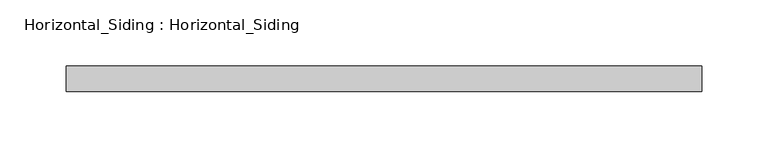
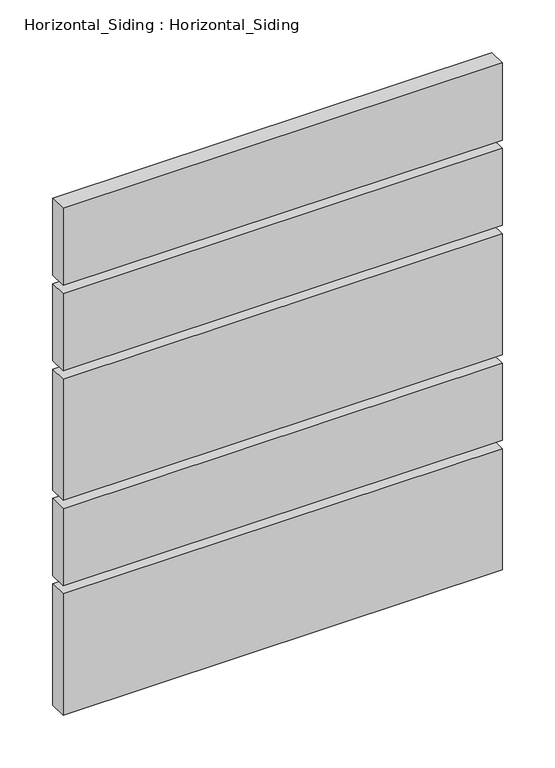
"""IFC4 building model written with IfcOpenShell, lengths in millimetres: plate geometry, Horizontal_Siding : Horizontal_Siding."""

from ifc_helpers import new_model, si_unit, frame, origin, place, context, project, spatial, polyline, outline, extrude, source, transform, mapped, element, save


def horizontal_siding_horizontal_siding_d49449ac(model_context):
    return source(origin(), model_context, "Body", "SweptSolid", [
        extrude(outline(polyline([(239.3754093, -19.05), (-239.3754093, -19.05), (-239.3754093, 0.0), (239.3754093, 0.0), (239.3754093, -19.05)])), frame((0.0, 0.0, 9.525), z_axis=(0.0, 0.0, 1.0), x_axis=(1.0, 0.0, 0.0)), (0.0, 0.0, 1.0), 139.7),
        extrude(outline(polyline([(239.3754093, -19.05), (-239.3754093, -19.05), (-239.3754093, 0.0), (239.3754093, 0.0), (239.3754093, -19.05)])), frame((0.0, 0.0, 158.75), z_axis=(0.0, 0.0, 1.0), x_axis=(1.0, 0.0, 0.0)), (0.0, 0.0, 1.0), 88.9),
        extrude(outline(polyline([(239.3754093, -19.05), (-239.3754093, -19.05), (-239.3754093, 0.0), (239.3754093, 0.0), (239.3754093, -19.05)])), frame((0.0, 0.0, 257.175), z_axis=(0.0, 0.0, 1.0), x_axis=(1.0, 0.0, 0.0)), (0.0, 0.0, 1.0), 139.7),
        extrude(outline(polyline([(239.3754093, -19.05), (-239.3754093, -19.05), (-239.3754093, 0.0), (239.3754093, 0.0), (239.3754093, -19.05)])), frame((0.0, 0.0, 406.4), z_axis=(0.0, 0.0, 1.0), x_axis=(1.0, 0.0, 0.0)), (0.0, 0.0, 1.0), 88.9),
        extrude(outline(polyline([(239.3754093, -19.05), (-239.3754093, -19.05), (-239.3754093, 0.0), (239.3754093, 0.0), (239.3754093, -19.05)])), frame((0.0, 0.0, 504.825), z_axis=(0.0, 0.0, 1.0), x_axis=(1.0, 0.0, 0.0)), (0.0, 0.0, 1.0), 88.9),
    ])


if __name__ == "__main__":
    model = new_model("IFC4")
    model_context = context("Model", 3, world=origin())
    ifc_project = project(units=[si_unit("LENGTHUNIT", "METRE", prefix="MILLI")], contexts=[model_context])
    site = spatial("IfcSite", under=ifc_project)
    building = spatial("IfcBuilding", under=site)
    placement = place(None, origin())
    horizontal_siding_horizontal_siding_shape = horizontal_siding_horizontal_siding_d49449ac(model_context)
    element("IfcPlate", 1, ObjectType="Horizontal_Siding : Horizontal_Siding", at=placement, inside=building, context=model_context, shape_type="MappedRepresentation", body=[
        mapped(horizontal_siding_horizontal_siding_shape, transform((0.0, 0.0, 0.0), x_axis=(1.0, 0.0, 0.0), y_axis=(0.0, 1.0, 0.0), z_axis=(0.0, 0.0, 1.0))),
    ])
    save(model, "model.ifc")

# Revit data of these elements
# Type "Horizontal_Siding : Horizontal_Siding"
#   Analytic Construction = "<None>"
#   extend = 0' - 2 3/4"
#   Width_2 = 0' - 3 1/2"
#   Width_1 = 0' - 5 1/2"
#   Gap = 0' - 0 3/8"
#   Plank Material = SLOTTED WOOD FENCE (THERMALLY MODIFIED WOOD: ARBOR WOOD)\n(EXTERIOR STAIN : PENOFIN VERDE EXT. STAIN - COLOR: CEDAR)
# Element 1 (IfcPlate, "Horizontal_Siding : Horizontal_Siding")
#   Materials on its faces: "SLOTTED WOOD FENCE (THERMALLY MODIFIED WOOD: ARBOR WOOD)\n(EXTERIOR STAIN : PENOFIN VERDE EXT. STAIN - COLOR: CEDAR)"
# Materials
#   "SLOTTED WOOD FENCE (THERMALLY MODIFIED WOOD: ARBOR WOOD)\n(EXTERIOR STAIN : PENOFIN VERDE EXT. STAIN - COLOR: CEDAR)": class "Wood", colour RGB 164 134 123, transparency 0, Description = "Pinus Echinata", Cost = 0
